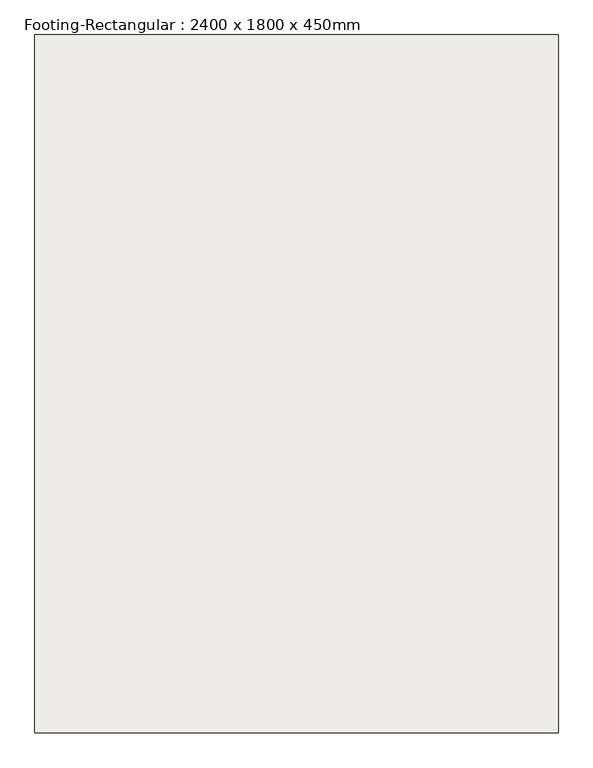
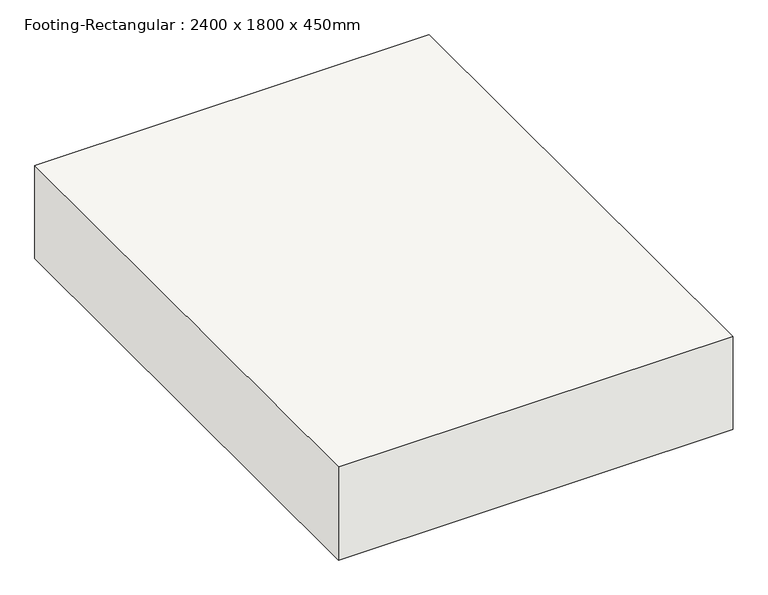
"""IFC4 building model written with IfcOpenShell, lengths in millimetres: slab geometry, Footing-Rectangular : 2400 x 1800 x 450mm."""

from ifc_helpers import new_model, si_unit, frame, origin, place, context, project, spatial, polyline, outline, extrude, source, transform, mapped, element, save


def footing_rectangular_2400_x_1800_x_450mm_039970dc(model_context):
    return source(origin(), model_context, "Body", "SweptSolid", [
        extrude(outline(polyline([(900.0, 1200.0), (900.0, -1200.0), (-900.0, -1200.0), (-900.0, 1200.0), (900.0, 1200.0)])), frame((0.0, 0.0, -450.0), z_axis=(0.0, 0.0, 1.0), x_axis=(1.0, 0.0, 0.0)), (0.0, 0.0, 1.0), 450.0),
    ])


if __name__ == "__main__":
    model = new_model("IFC4")
    model_context = context("Model", 3, world=origin())
    ifc_project = project(units=[si_unit("LENGTHUNIT", "METRE", prefix="MILLI")], contexts=[model_context])
    site = spatial("IfcSite", under=ifc_project)
    building = spatial("IfcBuilding", under=site)
    placement = place(None, origin())
    footing_rectangular_2400_x_1800_x_450mm_shape = footing_rectangular_2400_x_1800_x_450mm_039970dc(model_context)
    element("IfcSlab", 1, ObjectType="Footing-Rectangular : 2400 x 1800 x 450mm", at=placement, inside=building, context=model_context, shape_type="MappedRepresentation", body=[
        mapped(footing_rectangular_2400_x_1800_x_450mm_shape, transform((0.0, 0.0, 0.0), x_axis=(1.0, 0.0, 0.0), y_axis=(0.0, 1.0, 0.0), z_axis=(0.0, 0.0, 1.0))),
    ])
    save(model, "model.ifc")

# Revit data of these elements
# Type "Footing-Rectangular : 2400 x 1800 x 450mm"
#   Width = 1800 mm
#   Length = 2400 mm
#   Foundation Thickness = 450 mm
#   Structural Material [instance default] = Concrete - Cast-in-Place Concrete
#   Assembly Code = ""
# Element 1 (IfcSlab, "Footing-Rectangular : 2400 x 1800 x 450mm")
#   Materials on its faces: "Concrete - Cast-in-Place Concrete"
# Materials
#   "Concrete - Cast-in-Place Concrete": class "Concrete", colour RGB 192 192 192, transparency 0, Cost = 0
